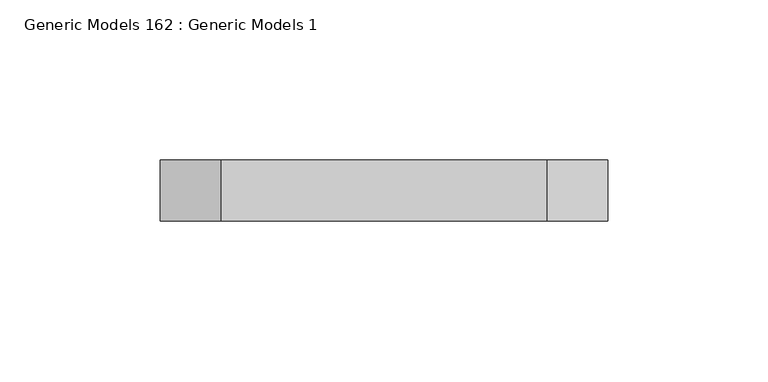
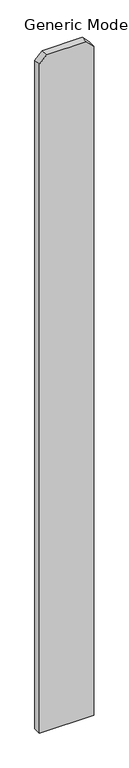
"""IFC4 building model written with IfcOpenShell, lengths in millimetres: proxy geometry, Generic Models 162 : Generic Models 1."""

from ifc_helpers import new_model, si_unit, frame, origin, place, context, project, spatial, polyline, outline, extrude, source, transform, mapped, element, save


def generic_models_162_generic_models_1_9f0ac15c(model_context):
    return source(origin(), model_context, "Body", "SweptSolid", [
        extrude(outline(polyline([(76.2, -250115.3875), (1885.95, -250115.3875), (1905.0, -250134.4375), (1905.0, -250236.0375), (1885.95, -250255.0875), (76.2, -250255.0875), (76.2, -250115.3875)])), frame((0.0, 547.6875, 0.0), z_axis=(0.0, 1.0, 0.0), x_axis=(0.0, 0.0, 1.0)), (0.0, 0.0, 1.0), 19.05),
    ])


if __name__ == "__main__":
    model = new_model("IFC4")
    model_context = context("Model", 3, world=origin())
    ifc_project = project(units=[si_unit("LENGTHUNIT", "METRE", prefix="MILLI")], contexts=[model_context])
    site = spatial("IfcSite", under=ifc_project)
    building = spatial("IfcBuilding", under=site)
    placement = place(None, origin())
    generic_models_162_generic_models_1_shape = generic_models_162_generic_models_1_9f0ac15c(model_context)
    element("IfcBuildingElementProxy", 1, Name="Generic Models 162 : Generic Models 1", ObjectType="Generic Models 162 : Generic Models 1", at=placement, inside=building, context=model_context, shape_type="MappedRepresentation", body=[
        mapped(generic_models_162_generic_models_1_shape, transform((0.0, 0.0, 0.0), x_axis=(1.0, 0.0, 0.0), y_axis=(0.0, 1.0, 0.0), z_axis=(0.0, 0.0, 1.0))),
    ])
    save(model, "model.ifc")

# Revit data of these elements
# Element 1 (IfcBuildingElementProxy, "Generic Models 162 : Generic Models 1")
#   Materials on its faces: "VERTICAL 1X6 CEDAR PLANKS W/ CLEAR WOOD SEALER"
# Materials
#   "VERTICAL 1X6 CEDAR PLANKS W/ CLEAR WOOD SEALER": class "Wood", colour RGB 234 198 147, transparency 0, Description = "Pinus Echinata", Cost = 0
